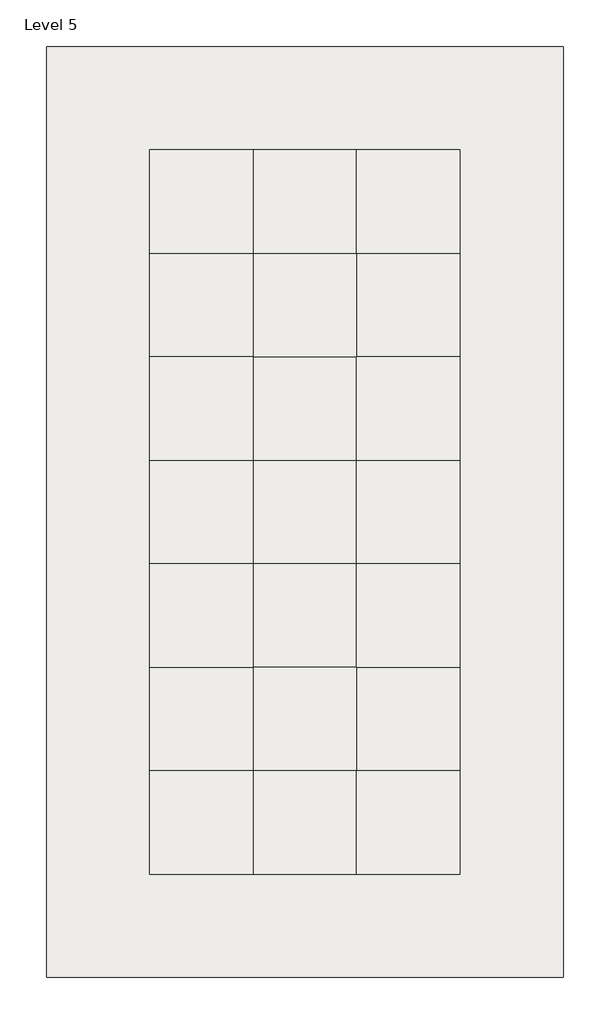
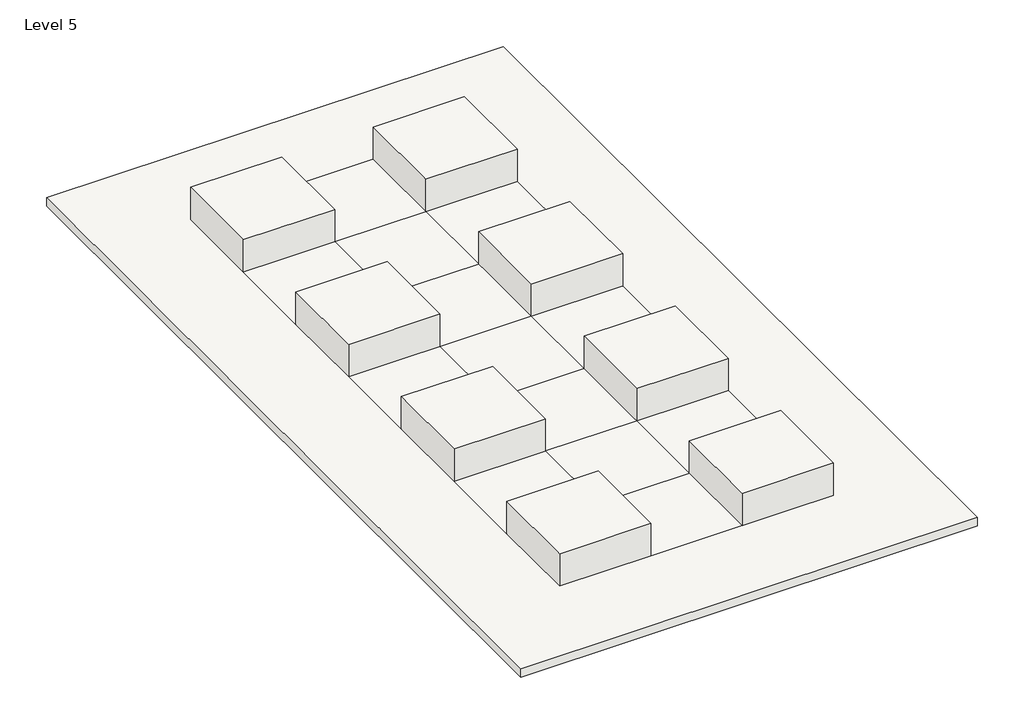
# One storey: 9 roofs.
"""IFC4 building model written with IfcOpenShell, lengths in millimetres."""

from ifc_helpers import new_model, si_unit, origin, place, context, project, spatial, faceted_brep, element, save

model = new_model("IFC4")

# Units and contexts
model_context = context("Model", 3, world=origin())
ifc_project = project(units=[si_unit("LENGTHUNIT", "METRE", prefix="MILLI")], contexts=[model_context])

# Site, building, storey
site = spatial("IfcSite", under=ifc_project)
building = spatial("IfcBuilding", under=site)
storey = spatial("IfcBuildingStorey", under=building, Name="Level 5", Elevation=20000.0)

# Roofs
placement = place(None, origin())
element("IfcRoof", 1, ObjectType="Bauder_RoofCoveringSystem_IntensiveGreenRoofSystem", at=placement, inside=storey, context=model_context, shape_type="Brep", body=[
    faceted_brep([(-674.7340554, 1676.2074539, 20000.0), (1325.2659446, 1676.2074539, 20000.0), (1325.2659446, -323.7925461, 20000.0), (-674.7340554, -323.7925461, 20000.0), (1325.2659446, 1676.2074539, 20949.8), (-674.7340554, 1676.2074539, 20949.8), (-674.7340554, -323.7925461, 20949.8), (1325.2659446, -323.7925461, 20949.8), (1325.2659446, 1676.2074539, 20200.0), (-674.7340554, 1676.2074539, 20200.0), (-674.7340554, -323.7925461, 20200.0), (1325.2659446, -323.7925461, 20200.0)], [[[0, 1, 2, 3]], [[4, 5, 6, 7]], [[5, 4, 8, 1, 0, 9]], [[6, 5, 9, 0, 3, 10]], [[7, 6, 10, 3, 2, 11]], [[4, 7, 11, 2, 1, 8]]]),
])
element("IfcRoof", 2, ObjectType="Bauder_RoofCoveringSystem_IntensiveGreenRoofSystem", at=placement, inside=storey, context=model_context, shape_type="Brep", body=[
    faceted_brep([(3325.2659446, 1676.2074539, 20000.0), (5325.2659446, 1676.2074539, 20000.0), (5325.2659446, -323.7925461, 20000.0), (3325.2659446, -323.7925461, 20000.0), (5325.2659446, 1676.2074539, 20949.8), (3325.2659446, 1676.2074539, 20949.8), (3325.2659446, -323.7925461, 20949.8), (5325.2659446, -323.7925461, 20949.8), (5325.2659446, 1676.2074539, 20200.0), (3325.2659446, 1676.2074539, 20200.0), (3325.2659446, -323.7925461, 20200.0), (5325.2659446, -323.7925461, 20200.0)], [[[0, 1, 2, 3]], [[4, 5, 6, 7]], [[5, 4, 8, 1, 0, 9]], [[6, 5, 9, 0, 3, 10]], [[7, 6, 10, 3, 2, 11]], [[4, 7, 11, 2, 1, 8]]]),
])
element("IfcRoof", 3, ObjectType="Bauder_RoofCoveringSystem_IntensiveGreenRoofSystem", at=placement, inside=storey, context=model_context, shape_type="Brep", body=[
    faceted_brep([(3325.2659446, -2323.7925461, 20000.0), (5325.2659446, -2323.7925461, 20000.0), (5325.2659446, -4323.7925461, 20000.0), (3325.2659446, -4323.7925461, 20000.0), (5325.2659446, -2323.7925461, 20949.8), (3325.2659446, -2323.7925461, 20949.8), (3325.2659446, -4323.7925461, 20949.8), (5325.2659446, -4323.7925461, 20949.8), (5325.2659446, -2323.7925461, 20200.0), (3325.2659446, -2323.7925461, 20200.0), (3325.2659446, -4323.7925461, 20200.0), (5325.2659446, -4323.7925461, 20200.0)], [[[0, 1, 2, 3]], [[4, 5, 6, 7]], [[5, 4, 8, 1, 0, 9]], [[6, 5, 9, 0, 3, 10]], [[7, 6, 10, 3, 2, 11]], [[4, 7, 11, 2, 1, 8]]]),
])
element("IfcRoof", 4, ObjectType="Bauder_RoofCoveringSystem_IntensiveGreenRoofSystem", at=placement, inside=storey, context=model_context, shape_type="Brep", body=[
    faceted_brep([(3325.2659446, -6323.7925461, 20000.0), (5325.2659446, -6323.7925461, 20000.0), (5325.2659446, -8323.7925461, 20000.0), (3325.2659446, -8323.7925461, 20000.0), (5325.2659446, -6323.7925461, 20949.8), (3325.2659446, -6323.7925461, 20949.8), (3325.2659446, -8323.7925461, 20949.8), (5325.2659446, -8323.7925461, 20949.8), (5325.2659446, -6323.7925461, 20200.0), (3325.2659446, -6323.7925461, 20200.0), (3325.2659446, -8323.7925461, 20200.0), (5325.2659446, -8323.7925461, 20200.0)], [[[0, 1, 2, 3]], [[4, 5, 6, 7]], [[5, 4, 8, 1, 0, 9]], [[6, 5, 9, 0, 3, 10]], [[7, 6, 10, 3, 2, 11]], [[4, 7, 11, 2, 1, 8]]]),
])
element("IfcRoof", 5, ObjectType="Bauder_RoofCoveringSystem_IntensiveGreenRoofSystem", at=placement, inside=storey, context=model_context, shape_type="Brep", body=[
    faceted_brep([(3325.2659446, -10323.7925461, 20000.0), (5325.2659446, -10323.7925461, 20000.0), (5325.2659446, -12323.7925461, 20000.0), (3325.2659446, -12323.7925461, 20000.0), (5325.2659446, -10323.7925461, 20949.8), (3325.2659446, -10323.7925461, 20949.8), (3325.2659446, -12323.7925461, 20949.8), (5325.2659446, -12323.7925461, 20949.8), (5325.2659446, -10323.7925461, 20200.0), (3325.2659446, -10323.7925461, 20200.0), (3325.2659446, -12323.7925461, 20200.0), (5325.2659446, -12323.7925461, 20200.0)], [[[0, 1, 2, 3]], [[4, 5, 6, 7]], [[5, 4, 8, 1, 0, 9]], [[6, 5, 9, 0, 3, 10]], [[7, 6, 10, 3, 2, 11]], [[4, 7, 11, 2, 1, 8]]]),
])
element("IfcRoof", 6, ObjectType="Bauder_RoofCoveringSystem_IntensiveGreenRoofSystem", at=placement, inside=storey, context=model_context, shape_type="Brep", body=[
    faceted_brep([(-674.7340554, -10323.7925461, 20000.0), (1325.2659446, -10323.7925461, 20000.0), (1325.2659446, -12323.7925461, 20000.0), (-674.7340554, -12323.7925461, 20000.0), (1325.2659446, -10323.7925461, 20949.8), (-674.7340554, -10323.7925461, 20949.8), (-674.7340554, -12323.7925461, 20949.8), (1325.2659446, -12323.7925461, 20949.8), (1325.2659446, -10323.7925461, 20200.0), (-674.7340554, -10323.7925461, 20200.0), (-674.7340554, -12323.7925461, 20200.0), (1325.2659446, -12323.7925461, 20200.0)], [[[0, 1, 2, 3]], [[4, 5, 6, 7]], [[5, 4, 8, 1, 0, 9]], [[6, 5, 9, 0, 3, 10]], [[7, 6, 10, 3, 2, 11]], [[4, 7, 11, 2, 1, 8]]]),
])
element("IfcRoof", 7, ObjectType="Bauder_RoofCoveringSystem_IntensiveGreenRoofSystem", at=placement, inside=storey, context=model_context, shape_type="Brep", body=[
    faceted_brep([(-674.7340554, -6323.7925461, 20000.0), (1325.2659446, -6323.7925461, 20000.0), (1325.2659446, -8323.7925461, 20000.0), (-674.7340554, -8323.7925461, 20000.0), (1325.2659446, -6323.7925461, 20949.8), (-674.7340554, -6323.7925461, 20949.8), (-674.7340554, -8323.7925461, 20949.8), (1325.2659446, -8323.7925461, 20949.8), (1325.2659446, -6323.7925461, 20200.0), (-674.7340554, -6323.7925461, 20200.0), (-674.7340554, -8323.7925461, 20200.0), (1325.2659446, -8323.7925461, 20200.0)], [[[0, 1, 2, 3]], [[4, 5, 6, 7]], [[5, 4, 8, 1, 0, 9]], [[6, 5, 9, 0, 3, 10]], [[7, 6, 10, 3, 2, 11]], [[4, 7, 11, 2, 1, 8]]]),
])
element("IfcRoof", 8, ObjectType="Bauder_RoofCoveringSystem_IntensiveGreenRoofSystem", at=placement, inside=storey, context=model_context, shape_type="Brep", body=[
    faceted_brep([(-674.7340554, -2323.7925461, 20000.0), (1325.2659446, -2323.7925461, 20000.0), (1325.2659446, -4323.7925461, 20000.0), (-674.7340554, -4323.7925461, 20000.0), (1325.2659446, -2323.7925461, 20949.8), (-674.7340554, -2323.7925461, 20949.8), (-674.7340554, -4323.7925461, 20949.8), (1325.2659446, -4323.7925461, 20949.8), (1325.2659446, -2323.7925461, 20200.0), (-674.7340554, -2323.7925461, 20200.0), (-674.7340554, -4323.7925461, 20200.0), (1325.2659446, -4323.7925461, 20200.0)], [[[0, 1, 2, 3]], [[4, 5, 6, 7]], [[5, 4, 8, 1, 0, 9]], [[6, 5, 9, 0, 3, 10]], [[7, 6, 10, 3, 2, 11]], [[4, 7, 11, 2, 1, 8]]]),
])
element("IfcRoof", 9, ObjectType="Roof_Concrete-200mm", at=placement, inside=storey, context=model_context, shape_type="Brep", body=[
    faceted_brep([(-2674.7340554, -14323.7925461, 20200.0), (-2674.7340554, -14323.7925461, 20000.0), (7325.2659446, -14323.7925461, 20000.0), (7325.2659446, -14323.7925461, 20200.0), (-2674.7340554, 3676.2074539, 20200.0), (-2674.7340554, 3676.2074539, 20000.0), (7325.2659446, 3676.2074539, 20200.0), (7325.2659446, 3676.2074539, 20000.0), (3325.2659446, 1676.2074539, 20200.0), (1325.2659446, 1676.2074539, 20200.0), (1325.2659446, -323.7925461, 20200.0), (3325.2659446, -323.7925461, 20200.0), (1325.2659446, 1676.2074539, 20000.0), (3325.2659446, 1676.2074539, 20000.0), (3325.2659446, -323.7925461, 20000.0), (1325.2659446, -323.7925461, 20000.0), (1325.2659446, -2323.7925461, 20200.0), (-674.7340554, -323.7925461, 20200.0), (-674.7340554, -2323.7925461, 20200.0), (3325.2659446, -2323.7925461, 20200.0), (5325.2659446, -2323.7925461, 20200.0), (5325.2659446, -323.7925461, 20200.0), (-674.7340554, -2323.7925461, 20000.0), (-674.7340554, -323.7925461, 20000.0), (1325.2659446, -2323.7925461, 20000.0), (3325.2659446, -2323.7925461, 20000.0), (5325.2659446, -323.7925461, 20000.0), (5325.2659446, -2323.7925461, 20000.0), (1325.2659446, -4323.7925461, 20200.0), (3325.2659446, -4323.7925461, 20200.0), (3325.2659446, -4323.7925461, 20000.0), (1325.2659446, -4323.7925461, 20000.0), (1325.2659446, -6323.7925461, 20200.0), (-674.7340554, -4323.7925461, 20200.0), (-674.7340554, -6323.7925461, 20200.0), (5325.2659446, -6323.7925461, 20200.0), (5325.2659446, -4323.7925461, 20200.0), (3325.2659446, -6323.7925461, 20200.0), (-674.7340554, -6323.7925461, 20000.0), (-674.7340554, -4323.7925461, 20000.0), (1325.2659446, -6323.7925461, 20000.0), (3325.2659446, -6323.7925461, 20000.0), (5325.2659446, -4323.7925461, 20000.0), (5325.2659446, -6323.7925461, 20000.0), (1325.2659446, -12323.7925461, 20200.0), (3325.2659446, -12323.7925461, 20200.0), (3325.2659446, -10323.7925461, 20200.0), (1325.2659446, -10323.7925461, 20200.0), (3325.2659446, -12323.7925461, 20000.0), (1325.2659446, -12323.7925461, 20000.0), (1325.2659446, -10323.7925461, 20000.0), (3325.2659446, -10323.7925461, 20000.0), (1325.2659446, -8323.7925461, 20200.0), (-674.7340554, -8323.7925461, 20200.0), (-674.7340554, -10323.7925461, 20200.0), (3325.2659446, -8323.7925461, 20200.0), (5325.2659446, -10323.7925461, 20200.0), (5325.2659446, -8323.7925461, 20200.0), (-674.7340554, -10323.7925461, 20000.0), (-674.7340554, -8323.7925461, 20000.0), (1325.2659446, -8323.7925461, 20000.0), (3325.2659446, -8323.7925461, 20000.0), (5325.2659446, -8323.7925461, 20000.0), (5325.2659446, -10323.7925461, 20000.0), (-674.7340554, 1676.2074539, 20000.0), (-674.7340554, 1676.2074539, 20200.0), (5325.2659446, 1676.2074539, 20200.0), (5325.2659446, 1676.2074539, 20000.0), (5325.2659446, -12323.7925461, 20000.0), (5325.2659446, -12323.7925461, 20200.0), (-674.7340554, -12323.7925461, 20000.0), (-674.7340554, -12323.7925461, 20200.0)], [[[0, 1, 2, 3]], [[1, 0, 4, 5]], [[6, 7, 5, 4]], [[3, 2, 7, 6]], [[8, 9, 10, 11]], [[12, 13, 14, 15]], [[16, 10, 17, 18]], [[11, 10, 16, 19]], [[20, 21, 11, 19]], [[22, 23, 15, 24]], [[15, 14, 25, 24]], [[25, 14, 26, 27]], [[19, 16, 28, 29]], [[24, 25, 30, 31]], [[32, 28, 33, 34]], [[35, 36, 29, 37]], [[38, 39, 31, 40]], [[41, 30, 42, 43]], [[44, 45, 46, 47]], [[48, 49, 50, 51]], [[47, 52, 53, 54]], [[47, 46, 55, 52]], [[56, 57, 55, 46]], [[58, 59, 60, 50]], [[51, 50, 60, 61]], [[51, 61, 62, 63]], [[52, 55, 37, 32]], [[29, 28, 32, 37]], [[61, 60, 40, 41]], [[31, 30, 41, 40]], [[9, 12, 15, 10]], [[10, 15, 23, 17]], [[17, 23, 64, 65]], [[12, 9, 65, 64]], [[66, 67, 26, 21]], [[21, 26, 14, 11]], [[11, 14, 13, 8]], [[67, 66, 8, 13]], [[20, 27, 42, 36]], [[36, 42, 30, 29]], [[29, 30, 25, 19]], [[27, 20, 19, 25]], [[16, 24, 31, 28]], [[28, 31, 39, 33]], [[33, 39, 22, 18]], [[24, 16, 18, 22]], [[32, 40, 60, 52]], [[52, 60, 59, 53]], [[53, 59, 38, 34]], [[40, 32, 34, 38]], [[35, 43, 62, 57]], [[57, 62, 61, 55]], [[55, 61, 41, 37]], [[43, 35, 37, 41]], [[56, 63, 68, 69]], [[69, 68, 48, 45]], [[45, 48, 51, 46]], [[63, 56, 46, 51]], [[47, 50, 49, 44]], [[44, 49, 70, 71]], [[71, 70, 58, 54]], [[50, 47, 54, 58]], [[4, 0, 3, 6], [9, 8, 66, 21, 20, 36, 35, 57, 56, 69, 45, 44, 71, 54, 53, 34, 33, 18, 17, 65]], [[7, 2, 1, 5], [13, 12, 64, 23, 22, 39, 38, 59, 58, 70, 49, 48, 68, 63, 62, 43, 42, 27, 26, 67]]]),
])

save(model, "model.ifc")

# Revit data of these elements
# Type "Bauder_RoofCoveringSystem_IntensiveGreenRoofSystem"
#   Keynote = "Q37"
#   Type IFC Predefined Type = "FLAT_ROOF"
#   Export Type to IFC As = "IfcRoofType"
#   Model = "Bauder Intensive Landscaping and Substrate - Intensive Green Roof System"
#   Manufacturer = "Bauder Ltd"
#   Type Comments = "Intensive Green Roof System"
#   URL = "http://www.bauder.co.uk/"
#   Description = "Bauder Intensive GreenRoof system incorporating Intensive Landscaping with Intensive Substrate, Filter Fleece, Mineral Drain, DSE60 Polyethylene Drainage and Protection Layer, FSM 1100 protection mat and PE Foil Polyethylene Separation-Slip Layer"
#   Assembly Code = "B3010"
#   NBSDescription = "Intensive green roof system"
#   NBSReference = "45-40-47/110"
#   BIMObjectName = "Bauder_RoofCoveringSystem_IntensiveGreenRoofSystem"
#   AccessibilityPerformance = "n/a"
#   CodePerformance = "n/a"
#   Color = "n/a"
#   Constituents = "n/a"
#   DurationUnit = "Year"
#   ExpectedLife = "n/a"
#   Features = "This BIM Object must be supported by a project specific specification from Bauder, incorporating system build-up, detail design and performance calculations if a full Bauder system guarantee is required. Please contact your local Bauder Representative or technical@bauder.co.uk"
#   Finish = "n/a"
#   Grade = "n/a"
#   Material = "n/a"
#   ModelReference = "Bauder Intensive Landscaping and Substrate - Intensive Green Roof System"
#   Name = "RoofCoveringSystem_Bauder_IntensiveGreenRoofSystem"
#   ReplacementCost = "n/a"
#   Shape = "n/a"
#   Size = "n/a"
#   SustainabilityPerformance = "Bauder Germany ISO14001: Certificate No.: 70499/03-15 e, Bauder UK ISO14001:Certificate No. 19ACM6595R, EN1271, BREEAM Credits Available"
#   WarrantyDescription = "Guarantee options could include ‘Product’, ‘Product and Workmanship’ and ‘Product, Workmanship and Design’ Guarantees. All guarantees available for this system are subject to the works being carried out in accordance with the Bauder specification and being installed by a Bauder Approved installer. For full details and further information regarding guarantees and alternative systems please contact your local Bauder Representative or technical@bauder.co.uk"
#   WarrantyDurationLabor = "n/a"
#   WarrantyDurationParts = "n/a\r\nn/a"
#   WarrantyDurationUnit = "Year"
#   WarrantyGuarantorLabor = "n/a"
#   WarrantyGuarantorParts = "technical@bauder.co.uk"
#   Certification = "n/a"
#   EdgeRestraints = "Perforated edge trim where required, refer to Bauder Project Specific Specification"
#   MoistureControlDrainageAncillaries = "n/a"
#   MoistureControlDrainageLayer = "Bauder DSE60 60 mm Polyethylene Drainage and Protection Layer with Bauder Mineral Drain Single size stone aggregate infill"
#   MoistureControlFilterMembrane = "Bauder Filter Fleece 1 mm Polypropylene Filter Fleece"
#   MoistureControlMoistureRetentionMat = "n/a"
#   PlantingSystemsAntierosionMat = "Jute Net where exposed, refer to Bauder Project Specific Specification"
#   PlantingSystemsPlantingMedium = "Bauder Intensive Substrate Recycled crushed brick, expanded clay shale and composted pine bark"
#   PlantingSystemsVegetation = "Bauder Intensive Landscaping"
#   PlantingSystemsVegetationBarrier = "20-40 mm Rounded-Washed Stones, refer to Bauder Project Specific Specification"
#   ProjectSpecificationAndDesign = "This BIM Object must be supported by a project specific specification from Bauder, incorporating system build-up, detail design and performance calculations if a full Bauder system warranty is required. Please contact your local Bauder Representative or technical@bauder.co.uk"
#   ProtectionProtectionLayer = "BauderGREEN FSM 1100 Protection Mat"
#   ProtectionRootBarrier = "As per project specific Bauder Specification"
#   ProtectionSeparationLayer = "2 layers of Bauder PE Foil 0.2 mm Polyethylene Separation-Slip Layer"
#   SystemManufacturer = "Bauder Ltd"
#   WarrantyConsiderations = "All guarantees available for this system are subject to the works being carried out in accordance with the Bauder specification and being installed by a Bauder Approved installer. For full details and further information regarding guarantees and alternative systems please contact your local Bauder Representative or technical@bauder.co.uk"
#   Update = "1900-12-31T23:59:59"
#   Documentation = "https://www.bauder.co.uk/technical-centre/technical-literature/system-brochures"
#   DocumentReference = "http://www.bauder.co.uk/"
#   IfcExportAs = "IfcRoofType"
#   IfcExportType = "FLAT_ROOF"
#   MethodOfMesurement = "n/a"
#   Process = "Replacement at service life intervals"
#   FireRating = "n/a"
#   _Author = "AM"
#   _AuthorizedBy = "bimstore"
#   _CreatedBy = "technical@bauder.co.uk"
#   _DistributedBy = "www.bimstore.co"
#   AssetType = "Fixed"
#   ClassificationName = "Uniclass2015"
#   ClassificationValue = "Ss_45_40_47_40"
#   CreatedBy = "technical@bauder.co.uk"
#   CreatedOn = "2023-02-10 T00:00:00"
#   DocumentationCertificates = "n/a"
#   DocumentationInstallationGuide = "https://www.bauder.co.uk/technical-centre"
#   DocumentationLiterature = "https://www.bauder.co.uk/technical-centre"
#   DocumentationMaintenance = "https://www.bauder.co.uk/technical-centre/maintenance-advice"
#   DocumentationTechnical = "https://www.bauder.co.uk/green-roofs/intensive-green-roofs"
#   ManufacturerName = "Bauder Ltd"
#   ModelNumber = "0910_INT-InS-FF-D6-F11-PE"
#   ProductionYear = "2023"
#   ReferencedStandard = "n/a"
#   SpareParts = "n/a"
#   TypeName = "Intensive Green Roof System"
#   NBSNote = "n/a"
#   NBSObjectName = "Bauder - Intensive green roof system"
#   NBSOfficeMasterTag = "n/a"
#   Ballast = "n/a"
#   CarrierMembraneFixing = "n/a"
#   CarrierMembraneType = "n/a"
#   FillToPerimeterUpstands = "n/a"
#   FilterLayer = "n/a"
#   InsulationFixing = "n/a"
#   InsulationType = "n/a"
#   LiquidAppliedWaterproofCoatingReinforcement = "n/a"
#   LiquidAppliedWaterproofCoatingSurfaceTreatment = "n/a"
#   LiquidAppliedWaterproofCoatingType = "n/a"
#   PreparationExistingSubstrates = "n/a"
#   PreparationHorizontalWork = "n/a"
#   PreparationSkirtingsAndVerticalWork = "n/a"
#   ProtectionLayer = "n/a"
#   SystemAccessories = "n/a"
#   WaterproofCoveringFirstLayerAttachment = "n/a"
#   WaterproofCoveringFirstLayerType = "n/a"
#   WaterproofCoveringIntermediateLayerAttachment = "n/a"
#   WaterproofCoveringIntermediateLayerType = "n/a"
#   WaterproofCoveringTopLayerAttachment = "n/a"
#   InsulationAttachment = "n/a"
#   IsolatingLayer = "n/a"
#   CarrierMembraneAttachment = "n/a"
#   LiquidAppliedWaterproofCoatingWearingCourse = "n/a"
#   VapourControlLayer = "n/a"
#   VapourControlLayerAttachment_Bauder = "n/a"
#   WaterproofCoveringJoints = "n/a"
#   WaterproofCoveringType = "n/a"
#   SeparatingLayer = "n/a"
#   WaterproofCoveringAccessories = "Yes"
#   WaterproofCoveringAttachment = "n/a"
#   UpperProtectionLayer = "n/a"
#   LowerProtectionLayer = "n/a"
#   WaterproofCoveringTopLayerType = "n/a"
#   DetailWorkAncillaryItems = "Detail as per project specific Bauder Specification"
#   DetailWorkCoverStrips = "Detail as per project specific Bauder Specification"
#   DetailWorkFlashings = "Detail as per project specific Bauder Specification"
#   DetailWorkSkirtingsAndUpstands = "Detail as per project specific Bauder Specification"
#   DetailWorkWeltedDrips = "Detail as per project specific Bauder Specification"
#   OverlayFixing = "n/a"
#   OverlayType = "n/a"
#   SurfaceProtection = "n/a"
#   VapourControlLayerAttachment = "n/a"
#   VapourControlLayerType = "n/a"
#   Cost = 0
#   NominalHeight = 0 mm
#   NominalLength = 0 mm
#   TotalArea = 0 m²
#   NominalDepth = 0 mm
#   IsExternal = yes
#   _BimSpecGuid = 0
#   _BSBibleVersion = 16
#   _CurrentRevision = 4
#   Layers, outside or top first: 300 mm "Bauder_Landscaping_Intensive" (function 5); 400 mm "Bauder_IntensiveSubstrate_BauderGREEN-SUB-IM-UK" (function 2); 1 mm "Bauder_FilterFleece_BauderGREEN-FV-125-100" (function 2); 40 mm "Bauder_DrainageBoard_BauderGREEN-DSE-40" (function 3); 8 mm "Bauder_ProtectionMat_BauderGREEN-FSM1100" (function 3); 200 mm "Concrete" (function 1); 0.8 mm "Bauder_SeparationAndSlipLayer_BauderGREEN-PE-02" (function 3)
# Type "Roof_Concrete-200mm"
#   Layers, outside or top first: 200 mm "Concrete" (function 1)
# Elements 1, 2, 3, 4, 5, 6, 7, 8 (IfcRoof, "Bauder_RoofCoveringSystem_IntensiveGreenRoofSystem")
#   built-in parameter 1001705 = 68.7329 (stored number, unit not read)
#   built-in parameter 1001710 = 33615
#   Phase Created = New Construction
#   Materials on its faces: "Bauder_SeparationAndSlipLayer_BauderGREEN-PE-02", "Bauder_Landscaping_Intensive"
# Element 9 (IfcRoof, "Roof_Concrete-200mm")
#   built-in parameter 1001710 = 33615
#   Phase Created = New Construction
#   Materials on its faces: "Concrete"
# Materials
#   "Bauder_Landscaping_Intensive": class "Unassigned", colour RGB 62 68 37, transparency 0, Mtrl_Author = "AM", Mtrl_AuthorizedBy = "bimstore", Mtrl_DistributedBy = "www.bimstore.co", Mtrl_AccessibilityPerformance = "n/a", Mtrl_AssetIdentifier = "Please record on commissioning", Mtrl_AssetType = "Fixed", Mtrl_BarCode = "Please record on commissioning", Mtrl_ClassificationName = "Uniclass2015", Mtrl_ClassificationValue = "n/a", Mtrl_CodePerformance = "n/a", Mtrl_Color = "n/a", Mtrl_Constituents = "n/a", Mtrl_CreatedBy = "technical@bauder.co.uk", Mtrl_CreatedOn = "2023-02-10 T00:00:00", Mtrl_DocumentationCertificates = "https://www.bimstore.co/products/intensive-green-roof-system/document/product-certificates", Mtrl_DocumentationInstallationGuide = "https://www.bimstore.co/products/intensive-green-roof-system/document/installation-guide", Mtrl_DocumentationLiterature = "https://www.bimstore.co/products/intensive-green-roof-system/document/product-literature", Mtrl_DocumentationMaintenance = "https://www.bimstore.co/products/intensive-green-roof-system/document/maintenance-information", Mtrl_DocumentationTechnical = "https://www.bimstore.co/products/intensive-green-roof-system/document/technical-data-sheet", Mtrl_DurationUnit = "Year", Mtrl_Features = "n/a", Mtrl_Finish = "n/a", Mtrl_Grade = "n/a", Mtrl_InstallationDate = "Please record on commissioning", Mtrl_ManufacturerName = "Bauder Ltd", Mtrl_Material = "n/a", Mtrl_ModelNumber = "Intensive", Mtrl_ModelReference = "Landscaping", Mtrl_ProductionYear = "2023", Mtrl_ReferencedStandard = "n/a", Mtrl_Shape = "n/a", Mtrl_Size = "n/a", Mtrl_SpareParts = "n/a", Mtrl_TypeName = "Intensive", Mtrl_WarrantyDescription = "n/a", Mtrl_WarrantyDurationUnit = "Year", Mtrl_WarrantyGuarantorLabor = "n/a", Mtrl_WarrantyGuarantorParts = "technical@bauder.co.uk", Mtrl_WarrantyStartDate = "Please record on commissioning", Mtrl_IfcExportAs = "IfcRoofType", Mtrl_IfcExportType = "FLAT_ROOF", Mtrl_BIMObjectName = "Bauder_Landscaping_Intensive", Mtrl_NBSDescription = "n/a", Mtrl_NBSNote = "n/a", Mtrl_NBSObjectName = "n/a", Mtrl_NBSOfficeMasterTag = "n/a", Mtrl_NBSReference = "Q37", Mtrl_Ballast = "n/a", Mtrl_CarrierMembraneAttachment = "n/a", Mtrl_CarrierMembraneFixing = "n/a", Mtrl_CarrierMembraneType = "n/a", Mtrl_Certification = "Comply with GRO Green Roof Code of Practice and FLL Standards", Mtrl_DetailWorkAncillaryItems = "Detail as per project specific Bauder Specification", Mtrl_DetailWorkCoverStrips = "Detail as per project specific Bauder Specification", Mtrl_DetailWorkFlashings = "Detail as per project specific Bauder Specification", Mtrl_DetailWorkSkirtingsAndUpstands = "Detail as per project specific Bauder Specification", Mtrl_DetailWorkWeltedDrips = "Detail as per project specific Bauder Specification", Mtrl_EdgeRestraints = "Detail as per project specific Bauder Specification", Mtrl_FillToPerimeterUpstands = "n/a", Mtrl_FilterLayer = "n/a", Mtrl_InsulationAttachment = "As per project specific Bauder Specification", Mtrl_InsulationFixing = "As per project specific Bauder Specification", Mtrl_InsulationType = "As per project specific Bauder Specification", Mtrl_IsolatingLayer = "n/a", Mtrl_LiquidAppliedWaterproofCoatingReinforcement = "n/a", Mtrl_LiquidAppliedWaterproofCoatingSurfaceTreatment = "As per project specific Bauder Specification", Mtrl_LiquidAppliedWaterproofCoatingType = "As per project specific Bauder Specification", Mtrl_LiquidAppliedWaterproofCoatingWearingCourse = "As per project specific Bauder Specification", Mtrl_LowerProtectionLayer = "n/a", Mtrl_MoistureControlDrainageAncillaries = "n/a", Mtrl_MoistureControlDrainageLayer = "n/a", Mtrl_MoistureControlFilterMembrane = "n/a", Mtrl_MoistureControlMoistureRetentionMat = "n/a", Mtrl_OverlayFixing = "n/a", Mtrl_OverlayType = "n/a", Mtrl_PlantingSystemsAntierosionMat = "n/a", Mtrl_PlantingSystemsPlantingMedium = "As per project specific Bauder Specification", Mtrl_PlantingSystemsVegetation = "As per project specific Bauder Specification", Mtrl_PlantingSystemsVegetationBarrier = "As per project specific Bauder Specification", Mtrl_PreparationExistingSubstrates = "n/a", Mtrl_PreparationHorizontalWork = "n/a", Mtrl_PreparationSkirtingsAndVerticalWork = "n/a", Mtrl_ProjectSpecificationAndDesign = "This BIM Object must be supported by a project specific specification from Bauder, incorporating system build-up, detail design and performance calculations if a full Bauder system warranty is required. Please contact your local Bauder Representative or technical@bauder.co.uk", Mtrl_ProtectionLayer = "n/a", Mtrl_ProtectionProtectionLayer = "n/a", Mtrl_ProtectionRootBarrier = "As per project specific Bauder Specification", Mtrl_ProtectionSeparationLayer = "n/a", Mtrl_SeparatingLayer = "n/a", Mtrl_SurfaceProtection = "n/a", Mtrl_SystemAccessories = "n/a", Mtrl_SystemManufacturer = "Bauder Ltd", Mtrl_Update = "1900-12-31 T23:59:59", Mtrl_UpperProtectionLayer = "n/a", Mtrl_VapourControlLayerAttachment = "As per project specific Bauder Specification", Mtrl_VapourControlLayerAttachment_Bauder = "As per project specific Bauder Specification", Mtrl_VapourControlLayerType = "As per project specific Bauder Specification", Mtrl_WarrantyConsiderations = "All guarantees available for this system are subject to the works being carried out in accordance with the Bauder specification and being installed by a Bauder Approved installer. For full details and further information regarding guarantees and alternative systems please contact your local Bauder Representative or technical@bauder.co.uk", Mtrl_WaterproofCoveringAccessories = "As per project specific Bauder Specification", Mtrl_WaterproofCoveringAttachment = "As per project specific Bauder Specification", Mtrl_WaterproofCoveringFirstLayerAttachment = "As per project specific Bauder Specification", Mtrl_WaterproofCoveringFirstLayerType = "As per project specific Bauder Specification", Mtrl_WaterproofCoveringIntermediateLayerAttachment = "As per project specific Bauder Specification", Mtrl_WaterproofCoveringIntermediateLayerType = "As per project specific Bauder Specification", Mtrl_WaterproofCoveringJoints = "As per project specific Bauder Specification", Mtrl_WaterproofCoveringTopLayerAttachment = "As per project specific Bauder Specification", Mtrl_WaterproofCoveringTopLayerType = "As per project specific Bauder Specification", Mtrl_WaterproofCoveringType = "As per project specific Bauder Specification", Cost = 0, Mtrl_ReplacementCost = 0, Mtrl_NominalDepth = 0 mm, Mtrl_NominalHeight = 0 mm, Mtrl_NominalLength = 0 mm, Mtrl_BimSpecGuid = 0, Mtrl_BSBibleVersion = 17, Mtrl_CurrentRevision = 2, Mtrl_ExpectedLife = 0, Mtrl_SerialNumber = 0, Mtrl_WarrantyDurationLabor = 0, Mtrl_WarrantyDurationParts = 0
#   "Bauder_IntensiveSubstrate_BauderGREEN-SUB-IM-UK": class "Unassigned", colour RGB 255 255 255, transparency 0, Mtrl_Author = "AM", Mtrl_AuthorizedBy = "bimstore", Mtrl_DistributedBy = "www.bimstore.co", Mtrl_AccessibilityPerformance = "n/a", Mtrl_AssetIdentifier = "Please record on commissioning", Mtrl_AssetType = "Fixed", Mtrl_BarCode = "Please record on commissioning", Mtrl_ClassificationName = "Uniclass2015", Mtrl_ClassificationValue = "n/a", Mtrl_CodePerformance = "n/a", Mtrl_Color = "n/a", Mtrl_Constituents = "n/a", Mtrl_CreatedBy = "technical@bauder.co.uk", Mtrl_CreatedOn = "2023-02-10 T00:00:00", Mtrl_DocumentationCertificates = "https://www.bimstore.co/products/intensive-green-roof-system/document/product-certificates", Mtrl_DocumentationInstallationGuide = "https://www.bimstore.co/products/intensive-green-roof-system/document/installation-guide", Mtrl_DocumentationLiterature = "https://www.bimstore.co/products/intensive-green-roof-system/document/product-literature", Mtrl_DocumentationMaintenance = "https://www.bimstore.co/products/intensive-green-roof-system/document/maintenance-information", Mtrl_DocumentationTechnical = "https://www.bimstore.co/products/intensive-green-roof-system/document/technical-data-sheet", Mtrl_DurationUnit = "Year", Mtrl_Features = "n/a", Mtrl_Finish = "n/a", Mtrl_Grade = "n/a", Mtrl_InstallationDate = "Please record on commissioning", Mtrl_ManufacturerName = "Bauder Ltd", Mtrl_Material = "Expanded Clay Aggregate", Mtrl_ModelNumber = "BauderGREEN-SUB-IM-UK", Mtrl_ModelReference = "Intensive Substrate", Mtrl_ProductionYear = "2023", Mtrl_ReferencedStandard = "n/a", Mtrl_Shape = "n/a", Mtrl_Size = "n/a", Mtrl_SpareParts = "n/a", Mtrl_TypeName = "BauderGREEN-SUB-IM-UK", Mtrl_WarrantyDescription = "As part of Bauder system guarantee, per specification", Mtrl_WarrantyDurationUnit = "Year", Mtrl_WarrantyGuarantorLabor = "n/a", Mtrl_WarrantyGuarantorParts = "technical@bauder.co.uk", Mtrl_WarrantyStartDate = "Please record on commissioning", Mtrl_IfcExportAs = "IfcRoofType", Mtrl_IfcExportType = "FLAT_ROOF", Mtrl_BIMObjectName = "Bauder_IntensiveSubstrate_BauderGREEN-SUB-IM-UK", Mtrl_NBSDescription = "n/a", Mtrl_NBSNote = "n/a", Mtrl_NBSObjectName = "n/a", Mtrl_NBSOfficeMasterTag = "n/a", Mtrl_NBSReference = "Q37", Mtrl_Ballast = "n/a", Mtrl_CarrierMembraneAttachment = "n/a", Mtrl_CarrierMembraneFixing = "n/a", Mtrl_CarrierMembraneType = "n/a", Mtrl_Certification = "Comply with GRO Green Roof Code of Practice and FLL Standards", Mtrl_DetailWorkAncillaryItems = "Detail as per project specific Bauder Specification", Mtrl_DetailWorkCoverStrips = "Detail as per project specific Bauder Specification", Mtrl_DetailWorkFlashings = "Detail as per project specific Bauder Specification", Mtrl_DetailWorkSkirtingsAndUpstands = "Detail as per project specific Bauder Specification", Mtrl_DetailWorkWeltedDrips = "Detail as per project specific Bauder Specification", Mtrl_EdgeRestraints = "Detail as per project specific Bauder Specification", Mtrl_FillToPerimeterUpstands = "n/a", Mtrl_FilterLayer = "n/a", Mtrl_InsulationAttachment = "As per project specific Bauder Specification", Mtrl_InsulationFixing = "As per project specific Bauder Specification", Mtrl_InsulationType = "As per project specific Bauder Specification", Mtrl_IsolatingLayer = "n/a", Mtrl_LiquidAppliedWaterproofCoatingReinforcement = "As per project specific Bauder Specification", Mtrl_LiquidAppliedWaterproofCoatingSurfaceTreatment = "As per project specific Bauder Specification", Mtrl_LiquidAppliedWaterproofCoatingType = "As per project specific Bauder Specification", Mtrl_LiquidAppliedWaterproofCoatingWearingCourse = "As per project specific Bauder Specification", Mtrl_LowerProtectionLayer = "n/a", Mtrl_MoistureControlDrainageAncillaries = "n/a", Mtrl_MoistureControlDrainageLayer = "n/a", Mtrl_MoistureControlFilterMembrane = "n/a", Mtrl_MoistureControlMoistureRetentionMat = "n/a", Mtrl_OverlayFixing = "n/a", Mtrl_OverlayType = "n/a", Mtrl_PlantingSystemsAntierosionMat = "n/a", Mtrl_PlantingSystemsPlantingMedium = "As per project specific Bauder Specification", Mtrl_PlantingSystemsVegetation = "As per project specific Bauder Specification", Mtrl_PlantingSystemsVegetationBarrier = "As per project specific Bauder Specification", Mtrl_PreparationExistingSubstrates = "n/a", Mtrl_PreparationHorizontalWork = "n/a", Mtrl_PreparationSkirtingsAndVerticalWork = "n/a", Mtrl_ProjectSpecificationAndDesign = "This BIM Object must be supported by a project specific specification from Bauder, incorporating system build-up, detail design and performance calculations if a full Bauder system warranty is required. Please contact your local Bauder Representative or technical@bauder.co.uk", Mtrl_ProtectionLayer = "n/a", Mtrl_ProtectionProtectionLayer = "n/a", Mtrl_ProtectionRootBarrier = "As per project specific Bauder Specification", Mtrl_ProtectionSeparationLayer = "n/a", Mtrl_SeparatingLayer = "n/a", Mtrl_SurfaceProtection = "n/a", Mtrl_SystemAccessories = "n/a", Mtrl_SystemManufacturer = "Bauder Ltd", Mtrl_Update = "1900-12-31 T23:59:59", Mtrl_UpperProtectionLayer = "n/a", Mtrl_VapourControlLayerAttachment = "As per project specific Bauder Specification", Mtrl_VapourControlLayerAttachment_Bauder = "As per project specific Bauder Specification", Mtrl_VapourControlLayerType = "As per project specific Bauder Specification", Mtrl_WarrantyConsiderations = "All guarantees available for this system are subject to the works being carried out in accordance with the Bauder specification and being installed by a Bauder Approved installer. For full details and further information regarding guarantees and alternative systems please contact your local Bauder Representative or technical@bauder.co.uk", Mtrl_WaterproofCoveringAccessories = "As per project specific Bauder Specification", Mtrl_WaterproofCoveringAttachment = "As per project specific Bauder Specification", Mtrl_WaterproofCoveringFirstLayerAttachment = "As per project specific Bauder Specification", Mtrl_WaterproofCoveringFirstLayerType = "As per project specific Bauder Specification", Mtrl_WaterproofCoveringIntermediateLayerAttachment = "As per project specific Bauder Specification", Mtrl_WaterproofCoveringIntermediateLayerType = "As per project specific Bauder Specification", Mtrl_WaterproofCoveringJoints = "As per project specific Bauder Specification", Mtrl_WaterproofCoveringTopLayerAttachment = "As per project specific Bauder Specification", Mtrl_WaterproofCoveringTopLayerType = "As per project specific Bauder Specification", Mtrl_WaterproofCoveringType = "As per project specific Bauder Specification", Cost = 0, Mtrl_ReplacementCost = 0, Mtrl_NominalDepth = 200 mm, Mtrl_NominalHeight = 0 mm, Mtrl_NominalLength = 0 mm, Mtrl_BimSpecGuid = 0, Mtrl_BSBibleVersion = 17, Mtrl_CurrentRevision = 2, Mtrl_ExpectedLife = 0, Mtrl_SerialNumber = 0, Mtrl_WarrantyDurationLabor = 0, Mtrl_WarrantyDurationParts = 0
#   "Bauder_FilterFleece_BauderGREEN-FV-125-100": class "Unassigned", colour RGB 255 255 255, transparency 0, Mtrl_Author = "AM", Mtrl_AuthorizedBy = "bimstore", Mtrl_DistributedBy = "www.bimstore.co", Mtrl_AccessibilityPerformance = "n/a", Mtrl_AssetIdentifier = "Please record on commissioning", Mtrl_AssetType = "Fixed", Mtrl_BarCode = "Please record on commissioning", Mtrl_ClassificationName = "Uniclass2015", Mtrl_ClassificationValue = "n/a", Mtrl_CodePerformance = "n/a", Mtrl_Color = "n/a", Mtrl_Constituents = "n/a", Mtrl_CreatedBy = "technical@bauder.co.uk", Mtrl_CreatedOn = "2023-02-10 T00:00:00", Mtrl_DocumentationCertificates = "https://www.bimstore.co/products/extensive-green-roof-system-wildflower-blanket/document/product-certificates", Mtrl_DocumentationInstallationGuide = "https://www.bimstore.co/products/extensive-green-roof-system-wildflower-blanket/document/installation-guide", Mtrl_DocumentationLiterature = "https://www.bimstore.co/products/intensive-green-roof-system/document/product-literature", Mtrl_DocumentationMaintenance = "https://www.bimstore.co/products/extensive-green-roof-system-wildflower-blanket/document/maintenance-information", Mtrl_DocumentationTechnical = "https://www.bimstore.co/products/extensive-green-roof-system-wildflower-blanket/document/technical-data-sheet", Mtrl_DurationUnit = "Year", Mtrl_Features = "n/a", Mtrl_Finish = "n/a", Mtrl_Grade = "n/a", Mtrl_InstallationDate = "Please record on commissioning", Mtrl_ManufacturerName = "Bauder Ltd", Mtrl_Material = "Polypropylene Fleece", Mtrl_ModelNumber = "BauderGREEN-FV-125-100", Mtrl_ModelReference = "Filter Fleece", Mtrl_ProductionYear = "2023", Mtrl_ReferencedStandard = "n/a", Mtrl_Shape = "n/a", Mtrl_Size = "n/a", Mtrl_SpareParts = "n/a", Mtrl_TypeName = "BauderGREEN-FV-125-100", Mtrl_WarrantyDescription = "As part of Bauder system guarantee, per specification", Mtrl_WarrantyDurationUnit = "Year", Mtrl_WarrantyGuarantorLabor = "technical@bauder.co.uk", Mtrl_WarrantyGuarantorParts = "technical@bauder.co.uk", Mtrl_WarrantyStartDate = "Please record on commissioning", Mtrl_IfcExportAs = "IfcRoofType", Mtrl_IfcExportType = "FLAT_ROOF", Mtrl_BIMObjectName = "Bauder_FilterFleece_BauderGREEN-FV-125-100", Mtrl_NBSDescription = "n/a", Mtrl_NBSNote = "n/a", Mtrl_NBSObjectName = "n/a", Mtrl_NBSOfficeMasterTag = "n/a", Mtrl_NBSReference = "Q37", Mtrl_Ballast = "n/a", Mtrl_CarrierMembraneAttachment = "n/a", Mtrl_CarrierMembraneFixing = "n/a", Mtrl_CarrierMembraneType = "n/a", Mtrl_Certification = "Comply with GRO Green Roof Code of Practice and FLL Standards", Mtrl_DetailWorkAncillaryItems = "Detail as per project specific Bauder Specification", Mtrl_DetailWorkCoverStrips = "Detail as per project specific Bauder Specification", Mtrl_DetailWorkFlashings = "Detail as per project specific Bauder Specification", Mtrl_DetailWorkSkirtingsAndUpstands = "Detail as per project specific Bauder Specification", Mtrl_DetailWorkWeltedDrips = "Detail as per project specific Bauder Specification", Mtrl_EdgeRestraints = "Detail as per project specific Bauder Specification", Mtrl_FillToPerimeterUpstands = "n/a", Mtrl_FilterLayer = "n/a", Mtrl_InsulationAttachment = "As per project specific Bauder Specification", Mtrl_InsulationFixing = "As per project specific Bauder Specification", Mtrl_InsulationType = "As per project specific Bauder Specification", Mtrl_IsolatingLayer = "n/a", Mtrl_LiquidAppliedWaterproofCoatingReinforcement = "As per project specific Bauder Specification", Mtrl_LiquidAppliedWaterproofCoatingSurfaceTreatment = "As per project specific Bauder Specification", Mtrl_LiquidAppliedWaterproofCoatingType = "As per project specific Bauder Specification", Mtrl_LiquidAppliedWaterproofCoatingWearingCourse = "As per project specific Bauder Specification", Mtrl_LowerProtectionLayer = "n/a", Mtrl_MoistureControlDrainageAncillaries = "n/a", Mtrl_MoistureControlDrainageLayer = "n/a", Mtrl_MoistureControlFilterMembrane = "n/a", Mtrl_MoistureControlMoistureRetentionMat = "n/a", Mtrl_OverlayFixing = "n/a", Mtrl_OverlayType = "n/a", Mtrl_PlantingSystemsAntierosionMat = "n/a", Mtrl_PlantingSystemsPlantingMedium = "As per project specific Bauder Specification", Mtrl_PlantingSystemsVegetation = "As per project specific Bauder Specification", Mtrl_PlantingSystemsVegetationBarrier = "As per project specific Bauder Specification", Mtrl_PreparationExistingSubstrates = "n/a", Mtrl_PreparationHorizontalWork = "n/a", Mtrl_PreparationSkirtingsAndVerticalWork = "n/a", Mtrl_ProjectSpecificationAndDesign = "This BIM Object must be supported by a project specific specification from Bauder, incorporating system build-up, detail design and performance calculations if a full Bauder system warranty is required. Please contact your local Bauder Representative or technical@bauder.co.uk", Mtrl_ProtectionLayer = "n/a", Mtrl_ProtectionProtectionLayer = "n/a", Mtrl_ProtectionRootBarrier = "As per project specific Bauder Specification", Mtrl_ProtectionSeparationLayer = "n/a", Mtrl_SeparatingLayer = "n/a", Mtrl_SurfaceProtection = "n/a", Mtrl_SystemAccessories = "n/a", Mtrl_SystemManufacturer = "Bauder Ltd", Mtrl_Update = "1900-12-31 T23:59:59", Mtrl_UpperProtectionLayer = "n/a", Mtrl_VapourControlLayerAttachment = "As per project specific Bauder Specification", Mtrl_VapourControlLayerAttachment_Bauder = "As per project specific Bauder Specification", Mtrl_VapourControlLayerType = "As per project specific Bauder Specification", Mtrl_WarrantyConsiderations = "All guarantees available for this system are subject to the works being carried out in accordance with the Bauder specification and being installed by a Bauder Approved installer. For full details and further information regarding guarantees and alternative systems please contact your local Bauder Representative or technical@bauder.co.uk", Mtrl_WaterproofCoveringAccessories = "As per project specific Bauder Specification", Mtrl_WaterproofCoveringAttachment = "As per project specific Bauder Specification", Mtrl_WaterproofCoveringFirstLayerAttachment = "As per project specific Bauder Specification", Mtrl_WaterproofCoveringFirstLayerType = "As per project specific Bauder Specification", Mtrl_WaterproofCoveringIntermediateLayerAttachment = "As per project specific Bauder Specification", Mtrl_WaterproofCoveringIntermediateLayerType = "As per project specific Bauder Specification", Mtrl_WaterproofCoveringJoints = "As per project specific Bauder Specification", Mtrl_WaterproofCoveringTopLayerAttachment = "As per project specific Bauder Specification", Mtrl_WaterproofCoveringTopLayerType = "As per project specific Bauder Specification", Mtrl_WaterproofCoveringType = "As per project specific Bauder Specification", Cost = 0, Mtrl_ReplacementCost = 0, Mtrl_NominalDepth = 1 mm, Mtrl_NominalHeight = 0 mm, Mtrl_NominalLength = 0 mm, Mtrl_BimSpecGuid = 0, Mtrl_BSBibleVersion = 17, Mtrl_CurrentRevision = 2, Mtrl_ExpectedLife = 0, Mtrl_SerialNumber = 0, Mtrl_WarrantyDurationLabor = 0, Mtrl_WarrantyDurationParts = 0
#   "Bauder_DrainageBoard_BauderGREEN-DSE-40": class "Unassigned", colour RGB 255 255 255, transparency 0, Mtrl_Author = "AM", Mtrl_AuthorizedBy = "bimstore", Mtrl_DistributedBy = "www.bimstore.co", Mtrl_AccessibilityPerformance = "n/a", Mtrl_AssetIdentifier = "Please record on commissioning", Mtrl_AssetType = "Fixed", Mtrl_BarCode = "Please record on commissioning", Mtrl_ClassificationName = "Uniclass2015", Mtrl_ClassificationValue = "Pr_65_67_78_72", Mtrl_CodePerformance = "n/a", Mtrl_Color = "n/a", Mtrl_Constituents = "n/a", Mtrl_CreatedBy = "technical@bauder.co.uk", Mtrl_CreatedOn = "2023-02-10 T00:00:00", Mtrl_DocumentationCertificates = "https://www.bimstore.co/products/extensive-green-roof-system-wildflower-blanket/document/product-certificates", Mtrl_DocumentationInstallationGuide = "https://www.bimstore.co/products/extensive-green-roof-system-wildflower-blanket/document/installation-guide", Mtrl_DocumentationLiterature = "https://www.bimstore.co/products/extensive-green-roof-system-wildflower-blanket/document/product-literature", Mtrl_DocumentationMaintenance = "https://www.bimstore.co/products/extensive-green-roof-system-wildflower-blanket/document/maintenance-information", Mtrl_DocumentationTechnical = "https://www.bimstore.co/products/extensive-green-roof-system-wildflower-blanket/document/technical-data-sheet", Mtrl_DurationUnit = "Year", Mtrl_Features = "n/a", Mtrl_Finish = "n/a", Mtrl_Grade = "n/a", Mtrl_InstallationDate = "Please record on commissioning", Mtrl_ManufacturerName = "Bauder Ltd", Mtrl_Material = "Recycled High Density Polyethylene", Mtrl_ModelNumber = "BauderGREEN-DSE-40", Mtrl_ModelReference = "Drainage Board", Mtrl_ProductionYear = "2023", Mtrl_ReferencedStandard = "n/a", Mtrl_Shape = "n/a", Mtrl_Size = "n/a", Mtrl_SpareParts = "n/a", Mtrl_TypeName = "BauderGREEN-DSE-40", Mtrl_WarrantyDescription = "As part of Bauder system guarantee, per specification", Mtrl_WarrantyDurationUnit = "Year", Mtrl_WarrantyGuarantorLabor = "technical@bauder.co.uk", Mtrl_WarrantyGuarantorParts = "technical@bauder.co.uk", Mtrl_WarrantyStartDate = "Please record on commissioning", Mtrl_IfcExportAs = "IfcRoofType", Mtrl_IfcExportType = "FLAT_ROOF", Mtrl_BIMObjectName = "Bauder_DrainageBoard_BauderGREEN-DSE-40", Mtrl_NBSDescription = "n/a", Mtrl_NBSNote = "n/a", Mtrl_NBSObjectName = "n/a", Mtrl_NBSOfficeMasterTag = "n/a", Mtrl_NBSReference = "Q37", Mtrl_Ballast = "n/a", Mtrl_CarrierMembraneAttachment = "n/a", Mtrl_CarrierMembraneFixing = "n/a", Mtrl_CarrierMembraneType = "n/a", Mtrl_Certification = "Comply with GRO Green Roof Code of Practice and FLL Standards", Mtrl_DetailWorkAncillaryItems = "Detail as per project specific Bauder Specification", Mtrl_DetailWorkCoverStrips = "Detail as per project specific Bauder Specification", Mtrl_DetailWorkFlashings = "Detail as per project specific Bauder Specification", Mtrl_DetailWorkSkirtingsAndUpstands = "Detail as per project specific Bauder Specification", Mtrl_DetailWorkWeltedDrips = "Detail as per project specific Bauder Specification", Mtrl_EdgeRestraints = "Detail as per project specific Bauder Specification", Mtrl_FillToPerimeterUpstands = "n/a", Mtrl_FilterLayer = "n/a", Mtrl_InsulationAttachment = "As per project specific Bauder Specification", Mtrl_InsulationFixing = "As per project specific Bauder Specification", Mtrl_InsulationType = "As per project specific Bauder Specification", Mtrl_IsolatingLayer = "n/a", Mtrl_LiquidAppliedWaterproofCoatingReinforcement = "As per project specific Bauder Specification", Mtrl_LiquidAppliedWaterproofCoatingSurfaceTreatment = "As per project specific Bauder Specification", Mtrl_LiquidAppliedWaterproofCoatingType = "As per project specific Bauder Specification", Mtrl_LiquidAppliedWaterproofCoatingWearingCourse = "As per project specific Bauder Specification", Mtrl_LowerProtectionLayer = "n/a", Mtrl_MoistureControlDrainageAncillaries = "n/a", Mtrl_MoistureControlDrainageLayer = "n/a", Mtrl_MoistureControlFilterMembrane = "n/a", Mtrl_MoistureControlMoistureRetentionMat = "n/a", Mtrl_OverlayFixing = "n/a", Mtrl_OverlayType = "n/a", Mtrl_PlantingSystemsAntierosionMat = "n/a", Mtrl_PlantingSystemsPlantingMedium = "As per project specific Bauder Specification", Mtrl_PlantingSystemsVegetation = "As per project specific Bauder Specification", Mtrl_PlantingSystemsVegetationBarrier = "As per project specific Bauder Specification", Mtrl_PreparationExistingSubstrates = "n/a", Mtrl_PreparationHorizontalWork = "n/a", Mtrl_PreparationSkirtingsAndVerticalWork = "n/a", Mtrl_ProjectSpecificationAndDesign = "This BIM Object must be supported by a project specific specification from Bauder, incorporating system build-up, detail design and performance calculations if a full Bauder system warranty is required. Please contact your local Bauder Representative or technical@bauder.co.uk", Mtrl_ProtectionLayer = "n/a", Mtrl_ProtectionProtectionLayer = "n/a", Mtrl_ProtectionRootBarrier = "As per project specific Bauder Specification", Mtrl_ProtectionSeparationLayer = "n/a", Mtrl_SeparatingLayer = "n/a", Mtrl_SurfaceProtection = "n/a", Mtrl_SystemAccessories = "n/a", Mtrl_SystemManufacturer = "Bauder Ltd", Mtrl_Update = "1900-12-31 T23:59:59", Mtrl_UpperProtectionLayer = "n/a", Mtrl_VapourControlLayerAttachment = "As per project specific Bauder Specification", Mtrl_VapourControlLayerAttachment_Bauder = "As per project specific Bauder Specification", Mtrl_VapourControlLayerType = "As per project specific Bauder Specification", Mtrl_WarrantyConsiderations = "All guarantees available for this system are subject to the works being carried out in accordance with the Bauder specification and being installed by a Bauder Approved installer. For full details and further information regarding guarantees and alternative systems please contact your local Bauder Representative or technical@bauder.co.uk", Mtrl_WaterproofCoveringAccessories = "As per project specific Bauder Specification", Mtrl_WaterproofCoveringAttachment = "As per project specific Bauder Specification", Mtrl_WaterproofCoveringFirstLayerAttachment = "As per project specific Bauder Specification", Mtrl_WaterproofCoveringFirstLayerType = "As per project specific Bauder Specification", Mtrl_WaterproofCoveringIntermediateLayerAttachment = "As per project specific Bauder Specification", Mtrl_WaterproofCoveringIntermediateLayerType = "As per project specific Bauder Specification", Mtrl_WaterproofCoveringJoints = "As per project specific Bauder Specification", Mtrl_WaterproofCoveringTopLayerAttachment = "As per project specific Bauder Specification", Mtrl_WaterproofCoveringTopLayerType = "As per project specific Bauder Specification", Mtrl_WaterproofCoveringType = "As per project specific Bauder Specification", Cost = 0, Mtrl_ReplacementCost = 0, Mtrl_NominalDepth = 40 mm, Mtrl_NominalHeight = 0 mm, Mtrl_NominalLength = 0 mm, Mtrl_BimSpecGuid = 0, Mtrl_BSBibleVersion = 17, Mtrl_CurrentRevision = 2, Mtrl_ExpectedLife = 0, Mtrl_SerialNumber = 0, Mtrl_WarrantyDurationLabor = 0, Mtrl_WarrantyDurationParts = 0
#   "Bauder_ProtectionMat_BauderGREEN-FSM1100": class "Unassigned", colour RGB 255 255 255, transparency 0, Mtrl_Author = "AM", Mtrl_AuthorizedBy = "bimstore", Mtrl_DistributedBy = "www.bimstore.co", Mtrl_AccessibilityPerformance = "n/a", Mtrl_AssetIdentifier = "Please record on commissioning", Mtrl_AssetType = "Fixed", Mtrl_BarCode = "Please record on commissioning", Mtrl_ClassificationName = "Uniclass2015", Mtrl_ClassificationValue = "Pr_20_96_71_64", Mtrl_CodePerformance = "n/a", Mtrl_Color = "n/a", Mtrl_Constituents = "n/a", Mtrl_CreatedBy = "technical@bauder.co.uk", Mtrl_CreatedOn = "2023-05-02 T00:00:00", Mtrl_DocumentationCertificates = "https://www.bimstore.co/products/intensive-green-roof-system/document/product-certificates", Mtrl_DocumentationInstallationGuide = "https://www.bimstore.co/products/intensive-green-roof-system/document/installation-guide", Mtrl_DocumentationLiterature = "https://www.bimstore.co/products/intensive-green-roof-system/document/product-literature", Mtrl_DocumentationMaintenance = "https://www.bimstore.co/products/intensive-green-roof-system/document/maintenance-information", Mtrl_DocumentationTechnical = "https://www.bimstore.co/products/intensive-green-roof-system/document/technical-data-sheet", Mtrl_DurationUnit = "Year", Mtrl_Features = "n/a", Mtrl_Finish = "n/a", Mtrl_Grade = "n/a", Mtrl_InstallationDate = "Please record on commissioning", Mtrl_ManufacturerName = "Bauder Ltd", Mtrl_Material = "Polyester and Polypropylene Fibre", Mtrl_ModelNumber = "BauderGREEN FSM1100", Mtrl_ModelReference = "Protection Mat", Mtrl_ProductionYear = "2023", Mtrl_ReferencedStandard = "n/a", Mtrl_Shape = "n/a", Mtrl_Size = "n/a", Mtrl_SpareParts = "n/a", Mtrl_TypeName = "BauderGREEN FSM1100", Mtrl_WarrantyDescription = "As part of Bauder system guarantee, per specification", Mtrl_WarrantyDurationUnit = "Year", Mtrl_WarrantyGuarantorLabor = "n/a", Mtrl_WarrantyGuarantorParts = "technical@bauder.co.uk", Mtrl_WarrantyStartDate = "Please record on commissioning", Mtrl_IfcExportAs = "IfcRoofType", Mtrl_IfcExportType = "FLAT_ROOF", Mtrl_BIMObjectName = "Bauder_ProtectionMat_BauderGREEN-FSM1100", Mtrl_NBSDescription = "n/a", Mtrl_NBSNote = "n/a", Mtrl_NBSObjectName = "n/a", Mtrl_NBSOfficeMasterTag = "n/a", Mtrl_NBSReference = "Q37", Mtrl_Ballast = "n/a", Mtrl_CarrierMembraneAttachment = "n/a", Mtrl_CarrierMembraneFixing = "n/a", Mtrl_CarrierMembraneType = "n/a", Mtrl_Certification = "Comply with GRO Green Roof Code of Practice and FLL Standards", Mtrl_DetailWorkAncillaryItems = "Detail as per project specific Bauder Specification", Mtrl_DetailWorkCoverStrips = "Detail as per project specific Bauder Specification", Mtrl_DetailWorkFlashings = "Detail as per project specific Bauder Specification", Mtrl_DetailWorkSkirtingsAndUpstands = "Detail as per project specific Bauder Specification", Mtrl_DetailWorkWeltedDrips = "Detail as per project specific Bauder Specification", Mtrl_EdgeRestraints = "Detail as per project specific Bauder Specification", Mtrl_FillToPerimeterUpstands = "n/a", Mtrl_FilterLayer = "n/a", Mtrl_InsulationAttachment = "As per project specific Bauder Specification", Mtrl_InsulationFixing = "As per project specific Bauder Specification", Mtrl_InsulationType = "As per project specific Bauder Specification", Mtrl_IsolatingLayer = "n/a", Mtrl_LiquidAppliedWaterproofCoatingReinforcement = "As per project specific Bauder Specification", Mtrl_LiquidAppliedWaterproofCoatingSurfaceTreatment = "As per project specific Bauder Specification", Mtrl_LiquidAppliedWaterproofCoatingType = "As per project specific Bauder Specification", Mtrl_LiquidAppliedWaterproofCoatingWearingCourse = "As per project specific Bauder Specification", Mtrl_LowerProtectionLayer = "n/a", Mtrl_MoistureControlDrainageAncillaries = "n/a", Mtrl_MoistureControlDrainageLayer = "n/a", Mtrl_MoistureControlFilterMembrane = "n/a", Mtrl_MoistureControlMoistureRetentionMat = "n/a", Mtrl_OverlayFixing = "n/a", Mtrl_OverlayType = "n/a", Mtrl_PlantingSystemsAntierosionMat = "n/a", Mtrl_PlantingSystemsPlantingMedium = "As per project specific Bauder Specification", Mtrl_PlantingSystemsVegetation = "As per project specific Bauder Specification", Mtrl_PlantingSystemsVegetationBarrier = "As per project specific Bauder Specification", Mtrl_PreparationExistingSubstrates = "n/a", Mtrl_PreparationHorizontalWork = "n/a", Mtrl_PreparationSkirtingsAndVerticalWork = "n/a", Mtrl_ProjectSpecificationAndDesign = "This BIM Object must be supported by a project specific specification from Bauder, incorporating system build-up, detail design and performance calculations if a full Bauder system warranty is required. Please contact your local Bauder Representative or technical@bauder.co.uk", Mtrl_ProtectionLayer = "n/a", Mtrl_ProtectionProtectionLayer = "n/a", Mtrl_ProtectionRootBarrier = "As per project specific Bauder Specification", Mtrl_ProtectionSeparationLayer = "n/a", Mtrl_SeparatingLayer = "n/a", Mtrl_SurfaceProtection = "n/a", Mtrl_SystemAccessories = "n/a", Mtrl_SystemManufacturer = "Bauder Ltd", Mtrl_Update = "1900-12-31 T23:59:59", Mtrl_UpperProtectionLayer = "n/a", Mtrl_VapourControlLayerAttachment = "As per project specific Bauder Specification", Mtrl_VapourControlLayerAttachment_Bauder = "As per project specific Bauder Specification", Mtrl_VapourControlLayerType = "As per project specific Bauder Specification", Mtrl_WarrantyConsiderations = "All guarantees available for this system are subject to the works being carried out in accordance with the Bauder specification and being installed by a Bauder Approved installer. For full details and further information regarding guarantees and alternative systems please contact your local Bauder Representative or technical@bauder.co.uk", Mtrl_WaterproofCoveringAccessories = "As per project specific Bauder Specification", Mtrl_WaterproofCoveringAttachment = "As per project specific Bauder Specification", Mtrl_WaterproofCoveringFirstLayerAttachment = "As per project specific Bauder Specification", Mtrl_WaterproofCoveringFirstLayerType = "As per project specific Bauder Specification", Mtrl_WaterproofCoveringIntermediateLayerAttachment = "As per project specific Bauder Specification", Mtrl_WaterproofCoveringIntermediateLayerType = "As per project specific Bauder Specification", Mtrl_WaterproofCoveringJoints = "As per project specific Bauder Specification", Mtrl_WaterproofCoveringTopLayerAttachment = "As per project specific Bauder Specification", Mtrl_WaterproofCoveringTopLayerType = "As per project specific Bauder Specification", Mtrl_WaterproofCoveringType = "As per project specific Bauder Specification", Cost = 0, Mtrl_ReplacementCost = 0, Mtrl_NominalDepth = 8 mm, Mtrl_NominalHeight = 0 mm, Mtrl_NominalLength = 0 mm, Mtrl_BimSpecGuid = 0, Mtrl_BSBibleVersion = 17, Mtrl_CurrentRevision = 2, Mtrl_ExpectedLife = 0, Mtrl_SerialNumber = 0, Mtrl_WarrantyDurationLabor = 0, Mtrl_WarrantyDurationParts = 0
#   "Concrete": class "Concrete", colour RGB 120 120 120, transparency 0, Description = "Portland Cement Concrete", Cost = 0
